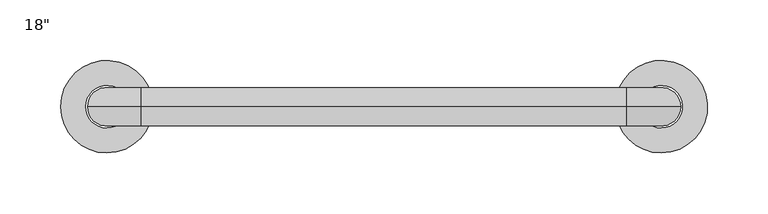
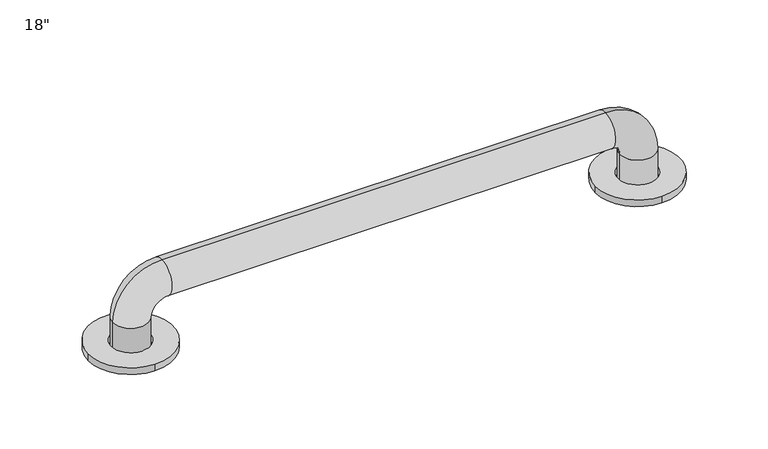
"""IFC4 building model written with IfcOpenShell, lengths in millimetres: proxy geometry."""

from ifc_helpers import new_model, si_unit, point, frame, frame_2d, origin, origin_with_axes, origin_2d, place, context, project, spatial, circle_curve, ellipse_curve, trimmed, segment, composite_curve, outline, extrude, source, transform, mapped, element, save
from ifc_brep_helpers import plane_surface, cylinder_surface, revolved_surface, advanced_brep


def proxy_9e031665(model_context):
    return source(origin(), model_context, "Body", "SolidModel", [
        extrude(outline(composite_curve([segment(trimmed(circle_curve(frame_2d((457.2, 0.0)), 38.1), [point((419.1, 0.0))], [point((457.2, -38.1))], False, "CARTESIAN"), True, "CONTINUOUS"), segment(trimmed(circle_curve(frame_2d((457.2, 0.0)), 38.1), [point((457.2, -38.1))], [point((419.1, 0.0))], False, "CARTESIAN"), True, "CONTINUOUS")], self_intersect=False), holes=[composite_curve([segment(trimmed(circle_curve(frame_2d((457.2, 0.0)), 17.4625), [point((439.7375, 0.0))], [point((457.2, -17.4625))], True, "CARTESIAN"), True, "CONTINUOUS"), segment(trimmed(circle_curve(frame_2d((457.2, 0.0)), 17.4625), [point((457.2, -17.4625))], [point((439.7375, 0.0))], True, "CARTESIAN"), True, "CONTINUOUS")], self_intersect=False)]), origin_with_axes(), (0.0, 0.0, 1.0), 6.35),
        extrude(outline(composite_curve([segment(trimmed(circle_curve(origin_2d(), 38.1), [point((-38.1, 0.0))], [point((0.0, -38.1))], False, "CARTESIAN"), True, "CONTINUOUS"), segment(trimmed(circle_curve(origin_2d(), 38.1), [point((0.0, -38.1))], [point((-38.1, 0.0))], False, "CARTESIAN"), True, "CONTINUOUS")], self_intersect=False), holes=[composite_curve([segment(trimmed(circle_curve(origin_2d(), 17.4625), [point((-17.4625, 0.0))], [point((0.0, -17.4625))], True, "CARTESIAN"), True, "CONTINUOUS"), segment(trimmed(circle_curve(origin_2d(), 17.4625), [point((0.0, -17.4625))], [point((-17.4625, 0.0))], True, "CARTESIAN"), True, "CONTINUOUS")], self_intersect=False)]), origin_with_axes(), (0.0, 0.0, 1.0), 6.35),
        advanced_brep(
        [(473.075, 0.0, 0.0), (441.325, 0.0, 0.0), (473.075, 0.0, 28.575), (441.325, 0.0, 28.575), (428.625, 0.0, 41.275), (428.625, 0.0, 73.025), (28.575, 0.0, 73.025), (28.575, 0.0, 41.275), (15.875, 0.0, 28.575), (-15.875, 0.0, 28.575), (-15.875, 0.0, 0.0), (15.875, 0.0, 0.0)],
        [
            (0, 1, circle_curve(frame((457.2, 0.0, 0.0), z_axis=(0.0, 0.0, -1.0), x_axis=(-1.0, 0.0, 0.0)), 15.875)),
            (1, 0, circle_curve(frame((457.2, 0.0, 0.0), z_axis=(0.0, 0.0, -1.0), x_axis=(-1.0, 0.0, 0.0)), 15.875)),
            (0, 2),
            (2, 3, circle_curve(frame((457.2, 0.0, 28.575), z_axis=(0.0, 0.0, -1.0), x_axis=(-1.0, 0.0, 0.0)), 15.875)),
            (3, 1),
            (3, 2, circle_curve(frame((457.2, 0.0, 28.575), z_axis=(0.0, 0.0, -1.0), x_axis=(-1.0, 0.0, 0.0)), 15.875)),
            (4, 3, circle_curve(frame((428.625, 0.0, 28.575), z_axis=(0.0, 1.0, 0.0), x_axis=(1.0, 0.0, 0.0)), 12.7)),
            (2, 5, circle_curve(frame((428.625, 0.0, 28.575), z_axis=(0.0, -1.0, 0.0), x_axis=(1.0, 0.0, 0.0)), 44.45)),
            (5, 4, circle_curve(frame((428.625, 0.0, 57.15), z_axis=(1.0, 0.0, 0.0), x_axis=(0.0, 0.0, -1.0)), 15.875)),
            (4, 5, circle_curve(frame((428.625, 0.0, 57.15), z_axis=(1.0, 0.0, 0.0), x_axis=(0.0, 0.0, -1.0)), 15.875)),
            (5, 6),
            (6, 7, circle_curve(frame((28.575, 0.0, 57.15), z_axis=(1.0, 0.0, 0.0), x_axis=(0.0, 0.0, -1.0)), 15.875)),
            (7, 4),
            (7, 6, circle_curve(frame((28.575, 0.0, 57.15), z_axis=(1.0, 0.0, 0.0), x_axis=(0.0, 0.0, -1.0)), 15.875)),
            (8, 7, circle_curve(frame((28.575, 0.0, 28.575), z_axis=(0.0, 1.0, 0.0), x_axis=(0.0, 0.0, 1.0)), 12.7)),
            (6, 9, circle_curve(frame((28.575, 0.0, 28.575), z_axis=(0.0, -1.0, 0.0), x_axis=(0.0, 0.0, 1.0)), 44.45)),
            (9, 8, circle_curve(frame((0.0, 0.0, 28.575), z_axis=(0.0, 0.0, 1.0), x_axis=(1.0, 0.0, 0.0)), 15.875)),
            (8, 9, circle_curve(frame((0.0, 0.0, 28.575), z_axis=(0.0, 0.0, 1.0), x_axis=(1.0, 0.0, 0.0)), 15.875)),
            (10, 11, circle_curve(frame((0.0, 0.0, 0.0), z_axis=(0.0, 0.0, -1.0), x_axis=(1.0, 0.0, 0.0)), 15.875)),
            (11, 10, circle_curve(frame((0.0, 0.0, 0.0), z_axis=(0.0, 0.0, -1.0), x_axis=(1.0, 0.0, 0.0)), 15.875)),
            (9, 10),
            (11, 8),
        ],
        [
            plane_surface(frame((457.2, 0.0, 0.0), z_axis=(0.0, 0.0, -1.0), x_axis=(0.0, -1.0, 0.0))),
            cylinder_surface(frame((457.2, 0.0, 0.0), z_axis=(0.0, 0.0, -1.0), x_axis=(-1.0, 0.0, 0.0)), 15.875),
            revolved_surface(trimmed(ellipse_curve(frame((457.2, 0.0, 28.575), z_axis=(0.0, 0.0, -1.0), x_axis=(-1.0, 0.0, 0.0)), 15.875, 15.875), [point((473.075, 0.0, 28.575))], [point((441.325, 0.0, 28.575))], True, "CARTESIAN"), (428.625, 0.0, 28.575), (0.0, -1.0, 0.0)),
            revolved_surface(trimmed(ellipse_curve(frame((457.2, 0.0, 28.575), z_axis=(0.0, 0.0, -1.0), x_axis=(-1.0, 0.0, 0.0)), 15.875, 15.875), [point((441.325, 0.0, 28.575))], [point((473.075, 0.0, 28.575))], True, "CARTESIAN"), (428.625, 0.0, 28.575), (0.0, -1.0, 0.0)),
            cylinder_surface(frame((428.625, 0.0, 57.15), z_axis=(1.0, 0.0, 0.0), x_axis=(0.0, 0.0, -1.0)), 15.875),
            revolved_surface(trimmed(ellipse_curve(frame((28.575, 0.0, 57.15), z_axis=(1.0, 0.0, 0.0), x_axis=(0.0, 0.0, -1.0)), 15.875, 15.875), [point((28.575, 0.0, 73.025))], [point((28.575, 0.0, 41.275))], True, "CARTESIAN"), (28.575, 0.0, 28.575), (0.0, -1.0, 0.0)),
            revolved_surface(trimmed(ellipse_curve(frame((28.575, 0.0, 57.15), z_axis=(1.0, 0.0, 0.0), x_axis=(0.0, 0.0, -1.0)), 15.875, 15.875), [point((28.575, 0.0, 41.275))], [point((28.575, 0.0, 73.025))], True, "CARTESIAN"), (28.575, 0.0, 28.575), (0.0, -1.0, 0.0)),
            plane_surface(frame((0.0, 0.0, 0.0), z_axis=(0.0, 0.0, -1.0), x_axis=(0.0, -1.0, 0.0))),
            cylinder_surface(frame((0.0, 0.0, 28.575), z_axis=(0.0, 0.0, 1.0), x_axis=(1.0, 0.0, 0.0)), 15.875),
        ],
        [
            (0, [[1, 2]]),
            (1, [[-1, 3, 4, 5]]),
            (1, [[-2, -5, 6, -3]]),
            (2, [[7, -4, 8, 9]]),
            (3, [[-8, -6, -7, 10]]),
            (4, [[-9, 11, 12, 13]]),
            (4, [[-10, -13, 14, -11]]),
            (5, [[15, -12, 16, 17]]),
            (6, [[-16, -14, -15, 18]]),
            (7, [[19, 20]]),
            (8, [[-17, 21, -20, 22]]),
            (8, [[-18, -22, -19, -21]]),
        ],
    ),
    ])


if __name__ == "__main__":
    model = new_model("IFC4")
    model_context = context("Model", 3, world=origin())
    ifc_project = project(units=[si_unit("LENGTHUNIT", "METRE", prefix="MILLI")], contexts=[model_context])
    site = spatial("IfcSite", under=ifc_project)
    building = spatial("IfcBuilding", under=site)
    placement = place(None, origin())
    proxy_shape = proxy_9e031665(model_context)
    element("IfcBuildingElementProxy", 1, Name="Seqm-Grab Bar : 18\"", ObjectType="Seqm-Grab Bar : 18\"", at=placement, inside=building, context=model_context, shape_type="MappedRepresentation", body=[
        mapped(proxy_shape, transform((0.0, 0.0, 0.0), x_axis=(1.0, 0.0, 0.0), y_axis=(0.0, 1.0, 0.0), z_axis=(0.0, 0.0, 1.0))),
    ])
    save(model, "model.ifc")

# Revit data of these elements
# Type "Seqm-Grab Bar : 18\""
#   Spec Number = "10 28 00"
#   Spec Description = "18\" GRAB BAR"
#   Length = 1' - 6"
#   Default Elevation = 4' - 0"
#   Grab Bar Material = GRAB BARS - AT ADA RESTROOMS ONLY
# Element 1 (IfcBuildingElementProxy, "Seqm-Grab Bar : 18\"")
#   Materials on its faces: "GRAB BARS - AT ADA RESTROOMS ONLY"
# Materials
#   "GRAB BARS - AT ADA RESTROOMS ONLY": class "Generic", colour RGB 120 120 120, transparency 0, Cost = 0
